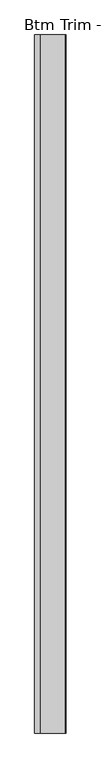
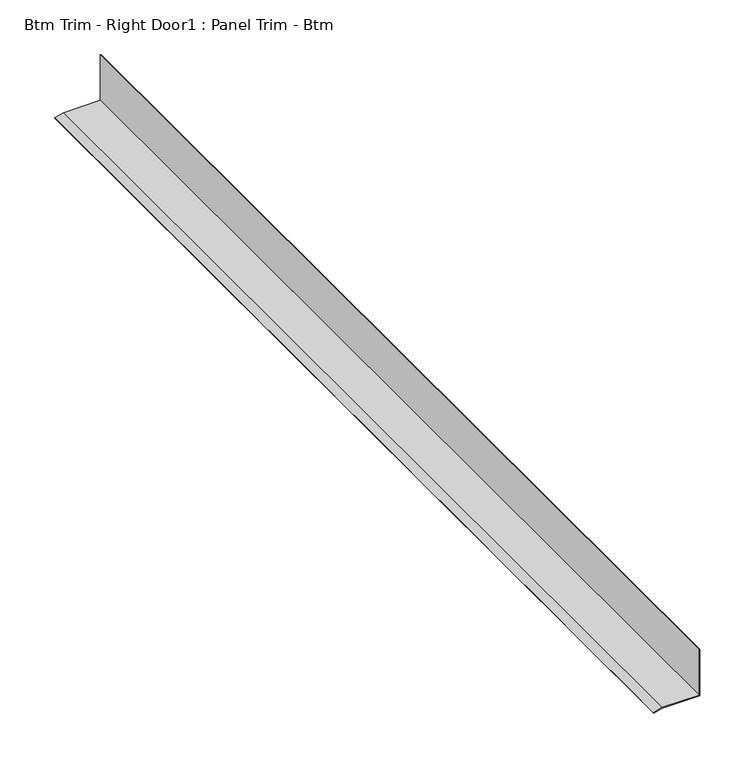
"""IFC4 building model written with IfcOpenShell, lengths in millimetres: proxy geometry, Btm Trim - Right Door1 : Panel Trim - Btm."""

from ifc_helpers import new_model, si_unit, frame, origin, place, context, project, spatial, polyline, outline, extrude, source, transform, mapped, element, save


def btm_trim_right_door1_panel_trim_btm_a276b19c(model_context):
    return source(origin(), model_context, "Body", "SweptSolid", [
        extrude(outline(polyline([(50.8, 587326.1141748), (48.3077022, 587316.8127928), (47.5409986, 587317.0182304), (50.00625, 587326.2186739), (50.00625, 587365.8934739), (101.6, 587365.8934739), (101.6, 587365.1060739), (50.8, 587365.1060739), (50.8, 587326.1141748)])), frame((0.0, -536301.7038841, 0.0), z_axis=(0.0, 1.0, 0.0), x_axis=(0.0, 0.0, 1.0)), (0.0, 0.0, 1.0), 1094.5749),
    ])


if __name__ == "__main__":
    model = new_model("IFC4")
    model_context = context("Model", 3, world=origin())
    ifc_project = project(units=[si_unit("LENGTHUNIT", "METRE", prefix="MILLI")], contexts=[model_context])
    site = spatial("IfcSite", under=ifc_project)
    building = spatial("IfcBuilding", under=site)
    placement = place(None, origin())
    btm_trim_right_door1_panel_trim_btm_shape = btm_trim_right_door1_panel_trim_btm_a276b19c(model_context)
    element("IfcBuildingElementProxy", 1, Name="Btm Trim - Right Door1 : Panel Trim - Btm", ObjectType="Btm Trim - Right Door1 : Panel Trim - Btm", at=placement, inside=building, context=model_context, shape_type="MappedRepresentation", body=[
        mapped(btm_trim_right_door1_panel_trim_btm_shape, transform((0.0, 0.0, 0.0), x_axis=(1.0, 0.0, 0.0), y_axis=(0.0, 1.0, 0.0), z_axis=(0.0, 0.0, 1.0))),
    ])
    save(model, "model.ifc")

# Revit data of these elements
# Element 1 (IfcBuildingElementProxy, "Btm Trim - Right Door1 : Panel Trim - Btm")
#   Materials on its faces: "BASE TRIM BY MTL PANEL MFR."
# Materials
#   "BASE TRIM BY MTL PANEL MFR.": class "Generic", colour RGB 239 242 240, transparency 0, Cost = 0
